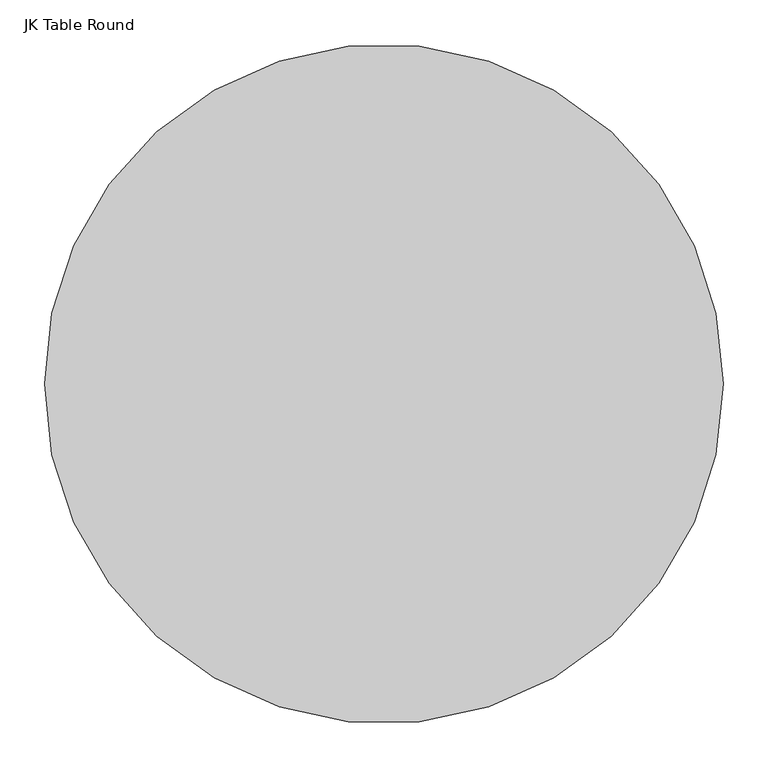
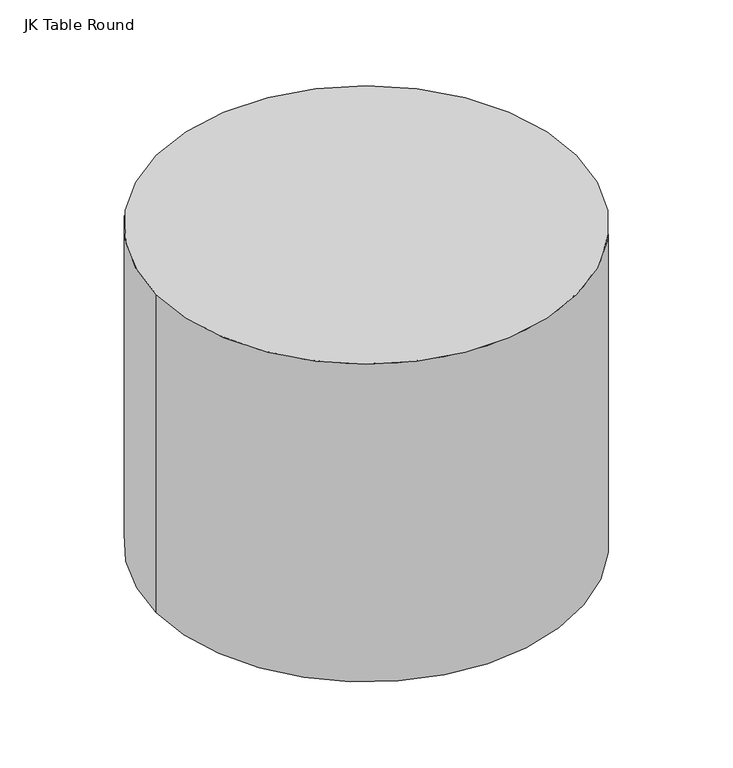
"""IFC4 building model written with IfcOpenShell, lengths in millimetres: furniture geometry, JK Table Round : DIC Endtable."""

import ifcopenshell
import ifcopenshell.guid

model = None  # the IFC model being written
_history = None  # IfcOwnerHistory: only IFC2X3 demands one
_inside = {}  # id of a spatial element -> (the spatial element, [elements in it])
_under = {}  # id of a project, library or spatial element -> (it, [spatial elements below it])
_declared = {}  # id of a project -> (the project, [libraries it declares])
_typed = {}  # id of a type object -> (the type object, [elements of that type])
_made_of = {}  # id of a material, layer set ... -> (it, [elements and type objects made of it])


def new_model(schema):
    """Start an empty IFC model of exactly this schema.

    Asked for "IFC4X3", IfcOpenShell would pick the latest addendum, in which some entities
    have other attributes; the version numbers below select the first issue.
    IFC2X3 requires an IfcOwnerHistory on every rooted entity: one is made here for all.
    """
    global model, _history
    if schema == "IFC4X3":
        model = ifcopenshell.file(schema_version=(4, 3, 0, 0))
    else:
        model = ifcopenshell.file(schema=schema)
    _inside.clear()
    _under.clear()
    _declared.clear()
    _typed.clear()
    _made_of.clear()
    _history = None
    if model.schema == "IFC2X3":
        org = make("IfcOrganization", Name="unknown")
        user = make(
            "IfcPersonAndOrganization",
            ThePerson=make("IfcPerson", FamilyName="unknown"),
            TheOrganization=org,
        )
        app = make(
            "IfcApplication",
            ApplicationDeveloper=org,
            Version="unknown",
            ApplicationFullName="unknown",
            ApplicationIdentifier="unknown",
        )
        _history = make(
            "IfcOwnerHistory",
            OwningUser=user,
            OwningApplication=app,
            ChangeAction="ADDED",
            CreationDate=0,
        )
    return model


def make(cls, **values):
    """One entity of the class cls with the attributes given. An attribute that is None is left unset."""
    return model.create_entity(
        cls, **{name: value for name, value in values.items() if value is not None}
    )


def rooted(cls, **values):
    """An entity with a GlobalId (a new one), such as an element, a storey or a relation."""
    return make(cls, GlobalId=ifcopenshell.guid.new(), OwnerHistory=_history, **values)


def si_unit(unit_type, name, prefix=None):
    """IfcSIUnit, for example si_unit("LENGTHUNIT", "METRE", prefix="MILLI")."""
    return make("IfcSIUnit", UnitType=unit_type, Prefix=prefix, Name=name)


def assignment(units):
    """IfcUnitAssignment: the units of a project."""
    return None if units is None else make("IfcUnitAssignment", Units=units)


def point(xyz):
    """IfcCartesianPoint."""
    return None if xyz is None else make("IfcCartesianPoint", Coordinates=xyz)


def direction(xyz):
    """IfcDirection."""
    return None if xyz is None else make("IfcDirection", DirectionRatios=xyz)


def frame(location, z_axis=None, x_axis=None):
    """IfcAxis2Placement3D, a coordinate frame: its origin and axes. An axis left out is left unset."""
    return make(
        "IfcAxis2Placement3D",
        Location=point(location),
        Axis=direction(z_axis),
        RefDirection=direction(x_axis),
    )


def frame_2d(location, x_axis=None):
    """IfcAxis2Placement2D, a coordinate frame in the plane: its origin and x axis."""
    return make(
        "IfcAxis2Placement2D", Location=point(location), RefDirection=direction(x_axis)
    )


def origin():
    """The frame at (0, 0, 0) with its axes left unset."""
    return frame((0.0, 0.0, 0.0))


def origin_with_axes():
    """The frame at (0, 0, 0) with the z axis (0, 0, 1) and the x axis (1, 0, 0) written out."""
    return frame((0.0, 0.0, 0.0), z_axis=(0.0, 0.0, 1.0), x_axis=(1.0, 0.0, 0.0))


def place(relative_to, where):
    """IfcLocalPlacement: puts the frame where relative to a parent placement (None: the world)."""
    return make(
        "IfcLocalPlacement", PlacementRelTo=relative_to, RelativePlacement=where
    )


def context(
    kind, dimensions, precision=None, world=None, true_north=None, identifier=None
):
    """IfcGeometricRepresentationContext, for example the 3D "Model" context."""
    return make(
        "IfcGeometricRepresentationContext",
        ContextIdentifier=identifier,
        ContextType=kind,
        CoordinateSpaceDimension=dimensions,
        Precision=precision,
        WorldCoordinateSystem=world,
        TrueNorth=true_north,
    )


def project(units=None, contexts=None):
    """IfcProject with its units and contexts."""
    return rooted(
        "IfcProject",
        Name="project",
        RepresentationContexts=contexts,
        UnitsInContext=assignment(units),
    )


def spatial(cls, under=None, at=None, **own):
    """A site, building, storey or space (cls), placed at a placement, below another one or the project."""
    s = rooted(cls, ObjectPlacement=at, **own)
    if under is not None:
        _under.setdefault(under.id(), (under, []))[1].append(s)
    return s


def circle_curve(where, radius):
    """IfcCircle in the frame where."""
    return make("IfcCircle", Position=where, Radius=radius)


def trimmed(basis, trim1, trim2, sense, master):
    """IfcTrimmedCurve: the piece of a basis curve between two trims."""
    return make(
        "IfcTrimmedCurve",
        BasisCurve=basis,
        Trim1=trim1,
        Trim2=trim2,
        SenseAgreement=sense,
        MasterRepresentation=master,
    )


def segment(curve, same_sense, transition):
    """IfcCompositeCurveSegment."""
    return make(
        "IfcCompositeCurveSegment",
        Transition=transition,
        SameSense=same_sense,
        ParentCurve=curve,
    )


def composite_curve(segments, self_intersect=None):
    """IfcCompositeCurve: segments joined end to end."""
    return make("IfcCompositeCurve", Segments=segments, SelfIntersect=self_intersect)


def outline(outer, holes=None, kind="AREA"):
    """IfcArbitraryClosedProfileDef: a profile drawn as a closed curve; with holes, ...WithVoids."""
    if holes is None:
        return make("IfcArbitraryClosedProfileDef", ProfileType=kind, OuterCurve=outer)
    return make(
        "IfcArbitraryProfileDefWithVoids",
        ProfileType=kind,
        OuterCurve=outer,
        InnerCurves=holes,
    )


def extrude(swept, where, along, depth):
    """IfcExtrudedAreaSolid: the profile swept, set in the frame where, extruded along a direction by depth."""
    return make(
        "IfcExtrudedAreaSolid",
        SweptArea=swept,
        Position=where,
        ExtrudedDirection=direction(along),
        Depth=depth,
    )


def shape(context_of_items, identifier, shape_type, items):
    """IfcShapeRepresentation: the items that make up one representation, for example the "Body"."""
    return make(
        "IfcShapeRepresentation",
        ContextOfItems=context_of_items,
        RepresentationIdentifier=identifier,
        RepresentationType=shape_type,
        Items=items,
    )


def source(mapping_origin, context_of_items, identifier, shape_type, items):
    """IfcRepresentationMap: a shape defined once, which mapped items show again and again."""
    return make(
        "IfcRepresentationMap",
        MappingOrigin=mapping_origin,
        MappedRepresentation=shape(context_of_items, identifier, shape_type, items),
    )


def transform(
    local_origin,
    x_axis=None,
    y_axis=None,
    z_axis=None,
    scale=None,
    scale2=None,
    scale3=None,
    uniform=True,
):
    """IfcCartesianTransformationOperator3D, or its non-uniform kind. x_axis, y_axis, z_axis: its Axis1, 2, 3."""
    if uniform:
        return make(
            "IfcCartesianTransformationOperator3D",
            Axis1=direction(x_axis),
            Axis2=direction(y_axis),
            LocalOrigin=point(local_origin),
            Scale=scale,
            Axis3=direction(z_axis),
        )
    return make(
        "IfcCartesianTransformationOperator3DnonUniform",
        Axis1=direction(x_axis),
        Axis2=direction(y_axis),
        LocalOrigin=point(local_origin),
        Scale=scale,
        Axis3=direction(z_axis),
        Scale2=scale2,
        Scale3=scale3,
    )


def mapped(mapping_source, mapping_target):
    """IfcMappedItem: shows the shape of a source again, moved by a transform."""
    return make(
        "IfcMappedItem", MappingSource=mapping_source, MappingTarget=mapping_target
    )


def made_of(thing, what):
    """Note that an element or type object is made of a material, layer set ...; save() writes the relation."""
    if what is not None:
        _made_of.setdefault(what.id(), (what, []))[1].append(thing)
    return thing


def element(
    cls,
    number,
    at=None,
    inside=None,
    cuts=None,
    type_object=None,
    material=None,
    context=None,
    identifier="Body",
    shape_type=None,
    held_by="IfcProductDefinitionShape",
    body=None,
    shapes=None,
    **own,
):
    """One element of the class cls, such as IfcWall. Its Tag is "e" and its number.

    at: its placement. inside: the storey or other place that contains it. cuts: it is an
    opening in that element (IfcRelVoidsElement). A single representation is given by context,
    identifier, shape_type and body (its items); several are given by shapes. held_by: the class
    of the entity that holds the representations. save() writes the other relations.
    """
    e = rooted(cls, Tag="e%d" % number, ObjectPlacement=at, **own)
    if body is not None:
        shapes = [shape(context, identifier, shape_type, body)]
    if shapes is not None:
        e.Representation = make(held_by, Representations=shapes)
    if inside is not None:
        _inside.setdefault(inside.id(), (inside, []))[1].append(e)
    if cuts is not None:
        rooted(
            "IfcRelVoidsElement", RelatingBuildingElement=cuts, RelatedOpeningElement=e
        )
    if type_object is not None:
        _typed.setdefault(type_object.id(), (type_object, []))[1].append(e)
    return made_of(e, material)


def aggregate(whole, parts):
    """IfcRelAggregates: a whole, such as a stair, and the parts it consists of."""
    return rooted("IfcRelAggregates", RelatingObject=whole, RelatedObjects=parts)


def save(model, path):
    """Write the relations noted so far, then the file.

    IfcRelAggregates (storeys below a building ...), IfcRelContainedInSpatialStructure (elements
    in a storey), IfcRelDefinesByType, IfcRelAssociatesMaterial and IfcRelDeclares: one each for
    every whole, place, type object, material and project.
    """
    for whole, parts in _under.values():
        aggregate(whole, parts)
    for where, things in _inside.values():
        rooted(
            "IfcRelContainedInSpatialStructure",
            RelatedElements=things,
            RelatingStructure=where,
        )
    for kind, things in _typed.values():
        rooted("IfcRelDefinesByType", RelatedObjects=things, RelatingType=kind)
    for what, things in _made_of.values():
        rooted("IfcRelAssociatesMaterial", RelatedObjects=things, RelatingMaterial=what)
    for by, libraries in _declared.values():
        rooted("IfcRelDeclares", RelatingContext=by, RelatedDefinitions=libraries)
    model.write(path)


def jk_table_round_730a3396(model_context):
    return source(origin(), model_context, "Body", "SweptSolid", [
        extrude(outline(composite_curve([segment(trimmed(circle_curve(frame_2d((-61.9426335, 33.5455296)), 381.0), [point((-442.9426335, 33.5455296))], [point((319.0573665, 33.5455296))], False, "CARTESIAN"), True, "CONTINUOUS"), segment(trimmed(circle_curve(frame_2d((-61.9426335, 33.5455296)), 381.0), [point((319.0573665, 33.5455296))], [point((-442.9426335, 33.5455296))], False, "CARTESIAN"), True, "CONTINUOUS")], self_intersect=False)), origin_with_axes(), (0.0, 0.0, 1.0), 609.6),
    ])


if __name__ == "__main__":
    model = new_model("IFC4")
    model_context = context("Model", 3, world=origin())
    ifc_project = project(units=[si_unit("LENGTHUNIT", "METRE", prefix="MILLI")], contexts=[model_context])
    site = spatial("IfcSite", under=ifc_project)
    building = spatial("IfcBuilding", under=site)
    placement = place(None, origin())
    jk_table_round_shape = jk_table_round_730a3396(model_context)
    element("IfcFurniture", 1, ObjectType="JK Table Round : DIC Endtable", at=placement, inside=building, context=model_context, shape_type="MappedRepresentation", body=[
        mapped(jk_table_round_shape, transform((0.0, 0.0, 0.0), x_axis=(1.0, 0.0, 0.0), y_axis=(0.0, 1.0, 0.0), z_axis=(0.0, 0.0, 1.0))),
    ])
    save(model, "model.ifc")

# Revit data of these elements
# Type "JK Table Round : DIC Endtable"
#   Width = 2' - 6"
#   Height = 2' - 0"
#   Status [instance default] = none
#   Default Elevation = 0
